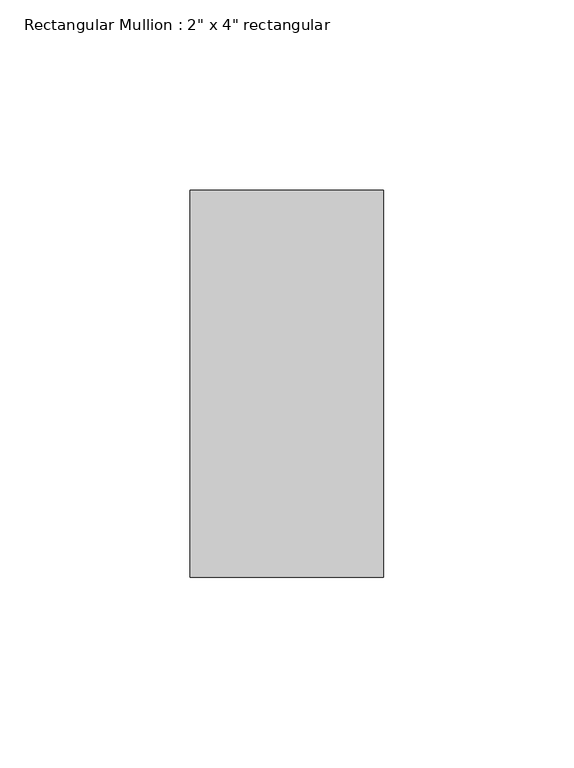
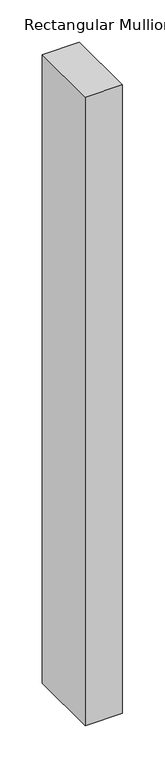
"""IFC4 building model written with IfcOpenShell, lengths in millimetres: member geometry."""

import ifcopenshell
import ifcopenshell.guid

model = None  # the IFC model being written
_history = None  # IfcOwnerHistory: only IFC2X3 demands one
_inside = {}  # id of a spatial element -> (the spatial element, [elements in it])
_under = {}  # id of a project, library or spatial element -> (it, [spatial elements below it])
_declared = {}  # id of a project -> (the project, [libraries it declares])
_typed = {}  # id of a type object -> (the type object, [elements of that type])
_made_of = {}  # id of a material, layer set ... -> (it, [elements and type objects made of it])


def new_model(schema):
    """Start an empty IFC model of exactly this schema.

    Asked for "IFC4X3", IfcOpenShell would pick the latest addendum, in which some entities
    have other attributes; the version numbers below select the first issue.
    IFC2X3 requires an IfcOwnerHistory on every rooted entity: one is made here for all.
    """
    global model, _history
    if schema == "IFC4X3":
        model = ifcopenshell.file(schema_version=(4, 3, 0, 0))
    else:
        model = ifcopenshell.file(schema=schema)
    _inside.clear()
    _under.clear()
    _declared.clear()
    _typed.clear()
    _made_of.clear()
    _history = None
    if model.schema == "IFC2X3":
        org = make("IfcOrganization", Name="unknown")
        user = make(
            "IfcPersonAndOrganization",
            ThePerson=make("IfcPerson", FamilyName="unknown"),
            TheOrganization=org,
        )
        app = make(
            "IfcApplication",
            ApplicationDeveloper=org,
            Version="unknown",
            ApplicationFullName="unknown",
            ApplicationIdentifier="unknown",
        )
        _history = make(
            "IfcOwnerHistory",
            OwningUser=user,
            OwningApplication=app,
            ChangeAction="ADDED",
            CreationDate=0,
        )
    return model


def make(cls, **values):
    """One entity of the class cls with the attributes given. An attribute that is None is left unset."""
    return model.create_entity(
        cls, **{name: value for name, value in values.items() if value is not None}
    )


def rooted(cls, **values):
    """An entity with a GlobalId (a new one), such as an element, a storey or a relation."""
    return make(cls, GlobalId=ifcopenshell.guid.new(), OwnerHistory=_history, **values)


def si_unit(unit_type, name, prefix=None):
    """IfcSIUnit, for example si_unit("LENGTHUNIT", "METRE", prefix="MILLI")."""
    return make("IfcSIUnit", UnitType=unit_type, Prefix=prefix, Name=name)


def assignment(units):
    """IfcUnitAssignment: the units of a project."""
    return None if units is None else make("IfcUnitAssignment", Units=units)


def point(xyz):
    """IfcCartesianPoint."""
    return None if xyz is None else make("IfcCartesianPoint", Coordinates=xyz)


def direction(xyz):
    """IfcDirection."""
    return None if xyz is None else make("IfcDirection", DirectionRatios=xyz)


def frame(location, z_axis=None, x_axis=None):
    """IfcAxis2Placement3D, a coordinate frame: its origin and axes. An axis left out is left unset."""
    return make(
        "IfcAxis2Placement3D",
        Location=point(location),
        Axis=direction(z_axis),
        RefDirection=direction(x_axis),
    )


def origin():
    """The frame at (0, 0, 0) with its axes left unset."""
    return frame((0.0, 0.0, 0.0))


def place(relative_to, where):
    """IfcLocalPlacement: puts the frame where relative to a parent placement (None: the world)."""
    return make(
        "IfcLocalPlacement", PlacementRelTo=relative_to, RelativePlacement=where
    )


def context(
    kind, dimensions, precision=None, world=None, true_north=None, identifier=None
):
    """IfcGeometricRepresentationContext, for example the 3D "Model" context."""
    return make(
        "IfcGeometricRepresentationContext",
        ContextIdentifier=identifier,
        ContextType=kind,
        CoordinateSpaceDimension=dimensions,
        Precision=precision,
        WorldCoordinateSystem=world,
        TrueNorth=true_north,
    )


def project(units=None, contexts=None):
    """IfcProject with its units and contexts."""
    return rooted(
        "IfcProject",
        Name="project",
        RepresentationContexts=contexts,
        UnitsInContext=assignment(units),
    )


def spatial(cls, under=None, at=None, **own):
    """A site, building, storey or space (cls), placed at a placement, below another one or the project."""
    s = rooted(cls, ObjectPlacement=at, **own)
    if under is not None:
        _under.setdefault(under.id(), (under, []))[1].append(s)
    return s


def polyline(points):
    """IfcPolyline through the points."""
    return make("IfcPolyline", Points=[point(p) for p in points])


def outline(outer, holes=None, kind="AREA"):
    """IfcArbitraryClosedProfileDef: a profile drawn as a closed curve; with holes, ...WithVoids."""
    if holes is None:
        return make("IfcArbitraryClosedProfileDef", ProfileType=kind, OuterCurve=outer)
    return make(
        "IfcArbitraryProfileDefWithVoids",
        ProfileType=kind,
        OuterCurve=outer,
        InnerCurves=holes,
    )


def extrude(swept, where, along, depth):
    """IfcExtrudedAreaSolid: the profile swept, set in the frame where, extruded along a direction by depth."""
    return make(
        "IfcExtrudedAreaSolid",
        SweptArea=swept,
        Position=where,
        ExtrudedDirection=direction(along),
        Depth=depth,
    )


def shape(context_of_items, identifier, shape_type, items):
    """IfcShapeRepresentation: the items that make up one representation, for example the "Body"."""
    return make(
        "IfcShapeRepresentation",
        ContextOfItems=context_of_items,
        RepresentationIdentifier=identifier,
        RepresentationType=shape_type,
        Items=items,
    )


def source(mapping_origin, context_of_items, identifier, shape_type, items):
    """IfcRepresentationMap: a shape defined once, which mapped items show again and again."""
    return make(
        "IfcRepresentationMap",
        MappingOrigin=mapping_origin,
        MappedRepresentation=shape(context_of_items, identifier, shape_type, items),
    )


def transform(
    local_origin,
    x_axis=None,
    y_axis=None,
    z_axis=None,
    scale=None,
    scale2=None,
    scale3=None,
    uniform=True,
):
    """IfcCartesianTransformationOperator3D, or its non-uniform kind. x_axis, y_axis, z_axis: its Axis1, 2, 3."""
    if uniform:
        return make(
            "IfcCartesianTransformationOperator3D",
            Axis1=direction(x_axis),
            Axis2=direction(y_axis),
            LocalOrigin=point(local_origin),
            Scale=scale,
            Axis3=direction(z_axis),
        )
    return make(
        "IfcCartesianTransformationOperator3DnonUniform",
        Axis1=direction(x_axis),
        Axis2=direction(y_axis),
        LocalOrigin=point(local_origin),
        Scale=scale,
        Axis3=direction(z_axis),
        Scale2=scale2,
        Scale3=scale3,
    )


def mapped(mapping_source, mapping_target):
    """IfcMappedItem: shows the shape of a source again, moved by a transform."""
    return make(
        "IfcMappedItem", MappingSource=mapping_source, MappingTarget=mapping_target
    )


def made_of(thing, what):
    """Note that an element or type object is made of a material, layer set ...; save() writes the relation."""
    if what is not None:
        _made_of.setdefault(what.id(), (what, []))[1].append(thing)
    return thing


def element(
    cls,
    number,
    at=None,
    inside=None,
    cuts=None,
    type_object=None,
    material=None,
    context=None,
    identifier="Body",
    shape_type=None,
    held_by="IfcProductDefinitionShape",
    body=None,
    shapes=None,
    **own,
):
    """One element of the class cls, such as IfcWall. Its Tag is "e" and its number.

    at: its placement. inside: the storey or other place that contains it. cuts: it is an
    opening in that element (IfcRelVoidsElement). A single representation is given by context,
    identifier, shape_type and body (its items); several are given by shapes. held_by: the class
    of the entity that holds the representations. save() writes the other relations.
    """
    e = rooted(cls, Tag="e%d" % number, ObjectPlacement=at, **own)
    if body is not None:
        shapes = [shape(context, identifier, shape_type, body)]
    if shapes is not None:
        e.Representation = make(held_by, Representations=shapes)
    if inside is not None:
        _inside.setdefault(inside.id(), (inside, []))[1].append(e)
    if cuts is not None:
        rooted(
            "IfcRelVoidsElement", RelatingBuildingElement=cuts, RelatedOpeningElement=e
        )
    if type_object is not None:
        _typed.setdefault(type_object.id(), (type_object, []))[1].append(e)
    return made_of(e, material)


def aggregate(whole, parts):
    """IfcRelAggregates: a whole, such as a stair, and the parts it consists of."""
    return rooted("IfcRelAggregates", RelatingObject=whole, RelatedObjects=parts)


def save(model, path):
    """Write the relations noted so far, then the file.

    IfcRelAggregates (storeys below a building ...), IfcRelContainedInSpatialStructure (elements
    in a storey), IfcRelDefinesByType, IfcRelAssociatesMaterial and IfcRelDeclares: one each for
    every whole, place, type object, material and project.
    """
    for whole, parts in _under.values():
        aggregate(whole, parts)
    for where, things in _inside.values():
        rooted(
            "IfcRelContainedInSpatialStructure",
            RelatedElements=things,
            RelatingStructure=where,
        )
    for kind, things in _typed.values():
        rooted("IfcRelDefinesByType", RelatedObjects=things, RelatingType=kind)
    for what, things in _made_of.values():
        rooted("IfcRelAssociatesMaterial", RelatedObjects=things, RelatingMaterial=what)
    for by, libraries in _declared.values():
        rooted("IfcRelDeclares", RelatingContext=by, RelatedDefinitions=libraries)
    model.write(path)


def member_0c09211d(model_context):
    return source(origin(), model_context, "Body", "SweptSolid", [
        extrude(outline(polyline([(25.4, 50.8), (25.4, -50.8), (-25.4, -50.8), (-25.4, 50.8), (25.4, 50.8)])), frame((0.0, 0.0, -907.1428571), z_axis=(0.0, 0.0, 1.0), x_axis=(1.0, 0.0, 0.0)), (0.0, 0.0, 1.0), 907.1428571),
    ])


if __name__ == "__main__":
    model = new_model("IFC4")
    model_context = context("Model", 3, world=origin())
    ifc_project = project(units=[si_unit("LENGTHUNIT", "METRE", prefix="MILLI")], contexts=[model_context])
    site = spatial("IfcSite", under=ifc_project)
    building = spatial("IfcBuilding", under=site)
    placement = place(None, origin())
    member_shape = member_0c09211d(model_context)
    element("IfcMember", 1, ObjectType="Rectangular Mullion : 2\" x 4\" rectangular", at=placement, inside=building, context=model_context, shape_type="MappedRepresentation", body=[
        mapped(member_shape, transform((0.0, 0.0, 0.0), x_axis=(1.0, 0.0, 0.0), y_axis=(0.0, 1.0, 0.0), z_axis=(0.0, 0.0, 1.0))),
    ])
    save(model, "model.ifc")

# Revit data of these elements
# Type "Rectangular Mullion : 2\" x 4\" rectangular"
#   built-in parameter 1007304 = 0.333333 (stored number, unit not read)
#   built-in parameter 1007301 = 0.0833333 (stored number, unit not read)
#   built-in parameter 1007300 = 0.0833333 (stored number, unit not read)
